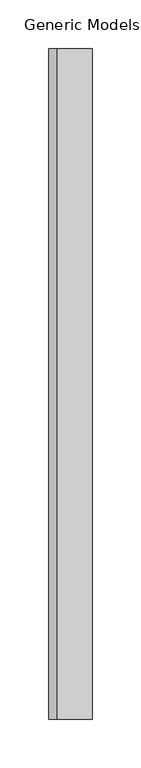
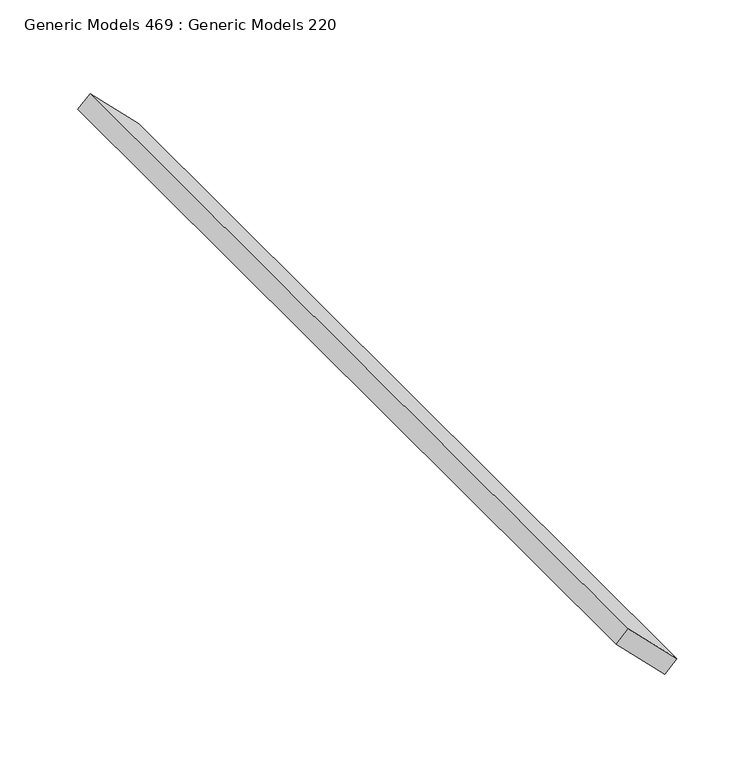
"""IFC4 building model written with IfcOpenShell, lengths in millimetres: proxy geometry, Generic Models 469 : Generic Models 220."""

from ifc_helpers import new_model, si_unit, frame, origin, place, context, project, spatial, polyline, outline, extrude, source, transform, mapped, element, save


def generic_models_469_generic_models_220_992a08f2(model_context):
    return source(origin(), model_context, "Body", "SweptSolid", [
        extrude(outline(polyline([(0.0, -50.8), (0.0, 0.0), (690.8142348, 0.0), (690.8142348, -50.8), (0.0, -50.8)])), frame((-6899.085451, -4564.8872686, 128196.1762561), z_axis=(0.7071067811865582, 0.0, 0.7071067811865369), x_axis=(0.0, 1.0, 0.0)), (0.0, 0.0, 1.0), 12.7),
    ])


if __name__ == "__main__":
    model = new_model("IFC4")
    model_context = context("Model", 3, world=origin())
    ifc_project = project(units=[si_unit("LENGTHUNIT", "METRE", prefix="MILLI")], contexts=[model_context])
    site = spatial("IfcSite", under=ifc_project)
    building = spatial("IfcBuilding", under=site)
    placement = place(None, origin())
    generic_models_469_generic_models_220_shape = generic_models_469_generic_models_220_992a08f2(model_context)
    element("IfcBuildingElementProxy", 1, Name="Generic Models 469 : Generic Models 220", ObjectType="Generic Models 469 : Generic Models 220", at=placement, inside=building, context=model_context, shape_type="MappedRepresentation", body=[
        mapped(generic_models_469_generic_models_220_shape, transform((0.0, 0.0, 0.0), x_axis=(1.0, 0.0, 0.0), y_axis=(0.0, 1.0, 0.0), z_axis=(0.0, 0.0, 1.0))),
    ])
    save(model, "model.ifc")

# Revit data of these elements
# Element 1 (IfcBuildingElementProxy, "Generic Models 469 : Generic Models 220")
#   Materials on its faces: "_WOOD TONE ALUMINUM EXTRUSION SLAT BY KNOTWOOD"
# Materials
#   "_WOOD TONE ALUMINUM EXTRUSION SLAT BY KNOTWOOD": class "Generic", colour RGB 177 130 114, transparency 0, Cost = 0
